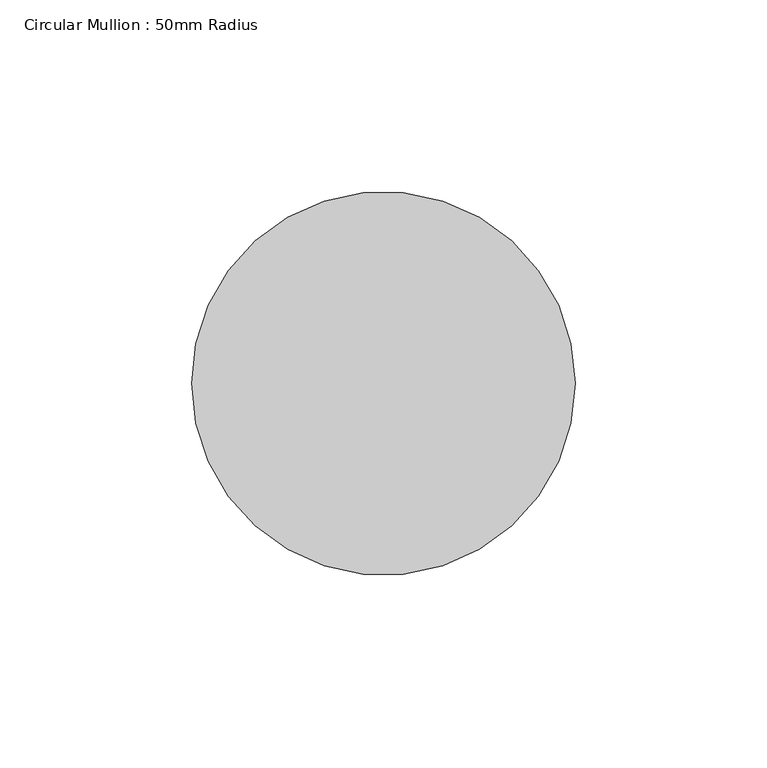
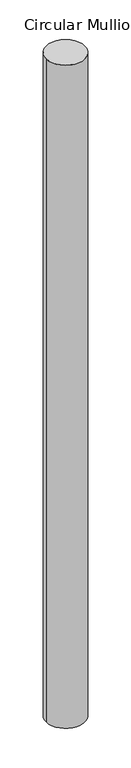
"""IFC4 building model written with IfcOpenShell, lengths in millimetres: member geometry, Circular Mullion : 50mm Radius."""

from ifc_helpers import new_model, si_unit, point, frame, origin, origin_2d, place, context, project, spatial, circle_curve, trimmed, segment, composite_curve, outline, extrude, source, transform, mapped, element, save


def circular_mullion_50mm_radius_bf84504b(model_context):
    return source(origin(), model_context, "Body", "SweptSolid", [
        extrude(outline(composite_curve([segment(trimmed(circle_curve(origin_2d(), 50.0), [point((50.0, 0.0))], [point((-50.0, 0.0))], False, "CARTESIAN"), True, "CONTINUOUS"), segment(trimmed(circle_curve(origin_2d(), 50.0), [point((-50.0, 0.0))], [point((50.0, 0.0))], False, "CARTESIAN"), True, "CONTINUOUS")], self_intersect=False)), frame((0.0, 0.0, -1810.8912097), z_axis=(0.0, 0.0, 1.0), x_axis=(1.0, 0.0, 0.0)), (0.0, 0.0, 1.0), 1810.8912097),
    ])


if __name__ == "__main__":
    model = new_model("IFC4")
    model_context = context("Model", 3, world=origin())
    ifc_project = project(units=[si_unit("LENGTHUNIT", "METRE", prefix="MILLI")], contexts=[model_context])
    site = spatial("IfcSite", under=ifc_project)
    building = spatial("IfcBuilding", under=site)
    placement = place(None, origin())
    circular_mullion_50mm_radius_shape = circular_mullion_50mm_radius_bf84504b(model_context)
    element("IfcMember", 1, ObjectType="Circular Mullion : 50mm Radius", at=placement, inside=building, context=model_context, shape_type="MappedRepresentation", body=[
        mapped(circular_mullion_50mm_radius_shape, transform((0.0, 0.0, 0.0), x_axis=(1.0, 0.0, 0.0), y_axis=(0.0, 1.0, 0.0), z_axis=(0.0, 0.0, 1.0))),
    ])
    save(model, "model.ifc")

# Revit data of these elements
# Type "Circular Mullion : 50mm Radius"
#   built-in parameter 1007350 = 0.164042 (stored number, unit not read)
# Element 1 (IfcMember, "Circular Mullion : 50mm Radius")
#   Materials on its faces: "Aluminium"
# Materials
#   "Aluminium": class "Metal", colour RGB 247 247 247, transparency 0, Description = "Aluminium 6061", Cost = 0
